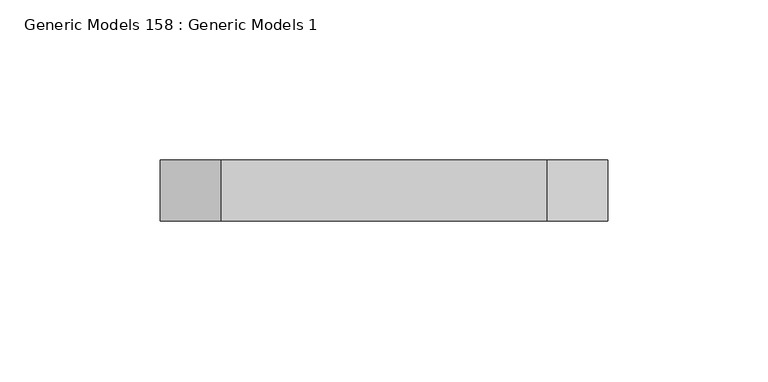
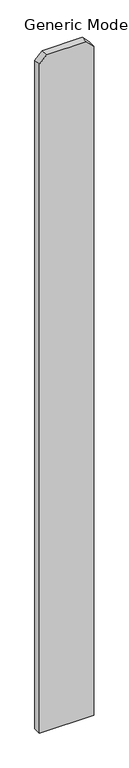
"""IFC4 building model written with IfcOpenShell, lengths in millimetres: proxy geometry, Generic Models 158 : Generic Models 1."""

from ifc_helpers import new_model, si_unit, frame, origin, place, context, project, spatial, polyline, outline, extrude, source, transform, mapped, element, save


def generic_models_158_generic_models_1_4ff7d1c7(model_context):
    return source(origin(), model_context, "Body", "SweptSolid", [
        extrude(outline(polyline([(76.2, 54075.0125), (1885.95, 54075.0125), (1905.0, 54055.9625), (1905.0, 53954.3625), (1885.95, 53935.3125), (76.2, 53935.3125), (76.2, 54075.0125)])), frame((0.0, 547.6875, 0.0), z_axis=(0.0, 1.0, 0.0), x_axis=(0.0, 0.0, 1.0)), (0.0, 0.0, 1.0), 19.05),
    ])


if __name__ == "__main__":
    model = new_model("IFC4")
    model_context = context("Model", 3, world=origin())
    ifc_project = project(units=[si_unit("LENGTHUNIT", "METRE", prefix="MILLI")], contexts=[model_context])
    site = spatial("IfcSite", under=ifc_project)
    building = spatial("IfcBuilding", under=site)
    placement = place(None, origin())
    generic_models_158_generic_models_1_shape = generic_models_158_generic_models_1_4ff7d1c7(model_context)
    element("IfcBuildingElementProxy", 1, Name="Generic Models 158 : Generic Models 1", ObjectType="Generic Models 158 : Generic Models 1", at=placement, inside=building, context=model_context, shape_type="MappedRepresentation", body=[
        mapped(generic_models_158_generic_models_1_shape, transform((0.0, 0.0, 0.0), x_axis=(1.0, 0.0, 0.0), y_axis=(0.0, 1.0, 0.0), z_axis=(0.0, 0.0, 1.0))),
    ])
    save(model, "model.ifc")

# Revit data of these elements
# Element 1 (IfcBuildingElementProxy, "Generic Models 158 : Generic Models 1")
#   Materials on its faces: "VERTICAL 1X6 CEDAR PLANKS W/ CLEAR WOOD SEALER"
# Materials
#   "VERTICAL 1X6 CEDAR PLANKS W/ CLEAR WOOD SEALER": class "Wood", colour RGB 234 198 147, transparency 0, Description = "Pinus Echinata", Cost = 0
